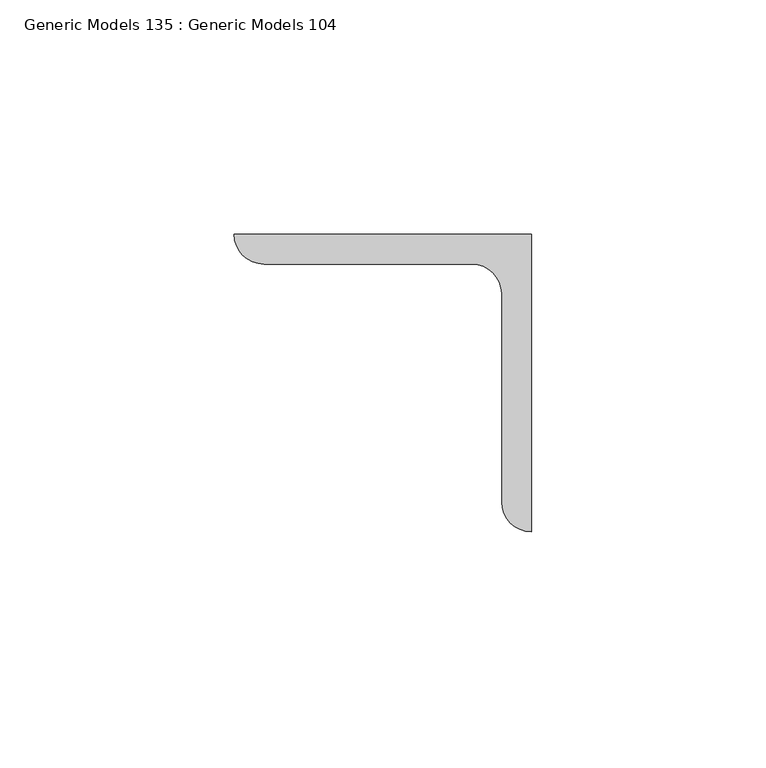
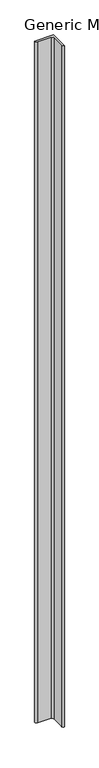
"""IFC4 building model written with IfcOpenShell, lengths in millimetres: proxy geometry, Generic Models 135 : Generic Models 104."""

from ifc_helpers import new_model, si_unit, point, frame, frame_2d, origin, place, context, project, spatial, polyline, circle_curve, trimmed, segment, composite_curve, outline, extrude, source, transform, mapped, element, save


def generic_models_135_generic_models_104_6f3c7f5b(model_context):
    return source(origin(), model_context, "Body", "SweptSolid", [
        extrude(outline(composite_curve([segment(polyline([(29176.0240778, 41071.1196612), (29176.0240778, 41007.6196612)]), True, "CONTINUOUS"), segment(trimmed(circle_curve(frame_2d((29176.0240778, 41013.9696612)), 6.35), [point((29176.0240778, 41007.6196612))], [point((29169.6740778, 41013.9696612))], False, "CARTESIAN"), True, "CONTINUOUS"), segment(polyline([(29169.6740778, 41013.9696612), (29169.6740778, 41058.4196612)]), True, "CONTINUOUS"), segment(trimmed(circle_curve(frame_2d((29163.3240778, 41058.4196612)), 6.35), [point((29169.6740778, 41058.4196612))], [point((29163.3240778, 41064.7696612))], True, "CARTESIAN"), True, "CONTINUOUS"), segment(polyline([(29163.3240778, 41064.7696612), (29118.8740778, 41064.7696612)]), True, "CONTINUOUS"), segment(trimmed(circle_curve(frame_2d((29118.8740778, 41071.1196612)), 6.35), [point((29118.8740778, 41064.7696612))], [point((29112.5240778, 41071.1196612))], False, "CARTESIAN"), True, "CONTINUOUS"), segment(polyline([(29112.5240778, 41071.1196612), (29176.0240778, 41071.1196612)]), True, "CONTINUOUS")], self_intersect=False)), frame((0.0, 0.0, 266407.9), z_axis=(0.0, 0.0, 1.0), x_axis=(1.0, 0.0, 0.0)), (0.0, 0.0, 1.0), 2432.1044757),
    ])


if __name__ == "__main__":
    model = new_model("IFC4")
    model_context = context("Model", 3, world=origin())
    ifc_project = project(units=[si_unit("LENGTHUNIT", "METRE", prefix="MILLI")], contexts=[model_context])
    site = spatial("IfcSite", under=ifc_project)
    building = spatial("IfcBuilding", under=site)
    placement = place(None, origin())
    generic_models_135_generic_models_104_shape = generic_models_135_generic_models_104_6f3c7f5b(model_context)
    element("IfcBuildingElementProxy", 1, Name="Generic Models 135 : Generic Models 104", ObjectType="Generic Models 135 : Generic Models 104", at=placement, inside=building, context=model_context, shape_type="MappedRepresentation", body=[
        mapped(generic_models_135_generic_models_104_shape, transform((0.0, 0.0, 0.0), x_axis=(1.0, 0.0, 0.0), y_axis=(0.0, 1.0, 0.0), z_axis=(0.0, 0.0, 1.0))),
    ])
    save(model, "model.ifc")

# Revit data of these elements
# Element 1 (IfcBuildingElementProxy, "Generic Models 135 : Generic Models 104")
#   Materials on its faces: "(2) BACK/BACK GALVANIZED ANGLES (2) L2 1/2 X 2 1/2 X 1/4\")"
# Materials
#   "(2) BACK/BACK GALVANIZED ANGLES (2) L2 1/2 X 2 1/2 X 1/4\")": class "Unassigned", colour RGB 211 211 211, transparency 0, Cost = 0
